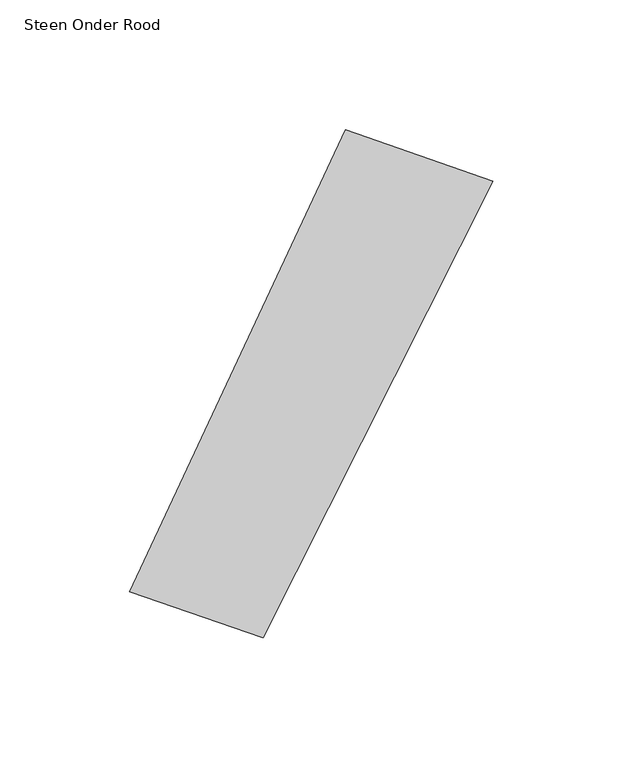
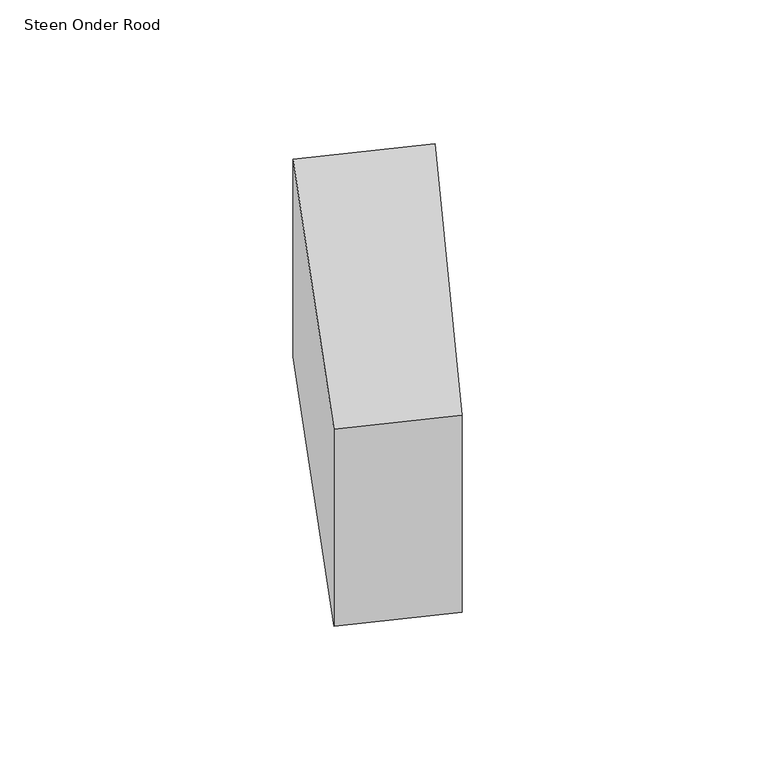
"""IFC4 building model written with IfcOpenShell, lengths in millimetres: proxy geometry, 00_GMA_steen_versie_4 : Steen Onder Rood."""

from ifc_helpers import new_model, si_unit, origin, origin_with_axes, place, context, project, spatial, polyline, outline, extrude, source, transform, mapped, element, save


def steen_onder_rood_f12f4f9c(model_context):
    return source(origin(), model_context, "Body", "SweptSolid", [
        extrude(outline(polyline([(143.9229616, 155.8712701), (55.4926521, -19.854313), (4.2117603, -1.9770767), (87.252236, 175.6122829), (143.9229616, 155.8712701)])), origin_with_axes(), (0.0, 0.0, 1.0), 100.0),
    ])


if __name__ == "__main__":
    model = new_model("IFC4")
    model_context = context("Model", 3, world=origin())
    ifc_project = project(units=[si_unit("LENGTHUNIT", "METRE", prefix="MILLI")], contexts=[model_context])
    site = spatial("IfcSite", under=ifc_project)
    building = spatial("IfcBuilding", under=site)
    placement = place(None, origin())
    steen_onder_rood_shape = steen_onder_rood_f12f4f9c(model_context)
    element("IfcBuildingElementProxy", 1, Name="00_GMA_steen_versie_4 : Steen Onder Rood", ObjectType="00_GMA_steen_versie_4 : Steen Onder Rood", at=placement, inside=building, context=model_context, shape_type="MappedRepresentation", body=[
        mapped(steen_onder_rood_shape, transform((0.0, 0.0, 0.0), x_axis=(1.0, 0.0, 0.0), y_axis=(0.0, 1.0, 0.0), z_axis=(0.0, 0.0, 1.0))),
    ])
    save(model, "model.ifc")

# Revit data of these elements
# Type "00_GMA_steen_versie_4 : Steen Onder Rood"
#   StootVoegHalfBoven [instance default] = 5 mm
#   StootVoegHalf [instance default] = 5 mm
#   StootVoegBreedteOnder = 10 mm
#   StootVoegBreedteBoven = 10 mm
#   Steendikte = 100 mm
#   LintVoegOnderHalf = 0 mm
#   LintVoegOnder = 0 mm
#   LintVoegBovenHalf = 5 mm
#   LintVoegBoven = 10 mm
#   materiaal = 21_steen_rood
#   MateriaalVoeg = none
#   Default Elevation = 0
# Element 1 (IfcBuildingElementProxy, "00_GMA_steen_versie_4 : Steen Onder Rood")
#   Materials on its faces: "21_steen_rood"
# Materials
#   "21_steen_rood": class "Unassigned", colour RGB 213 111 43, transparency 0, Cost = 0
